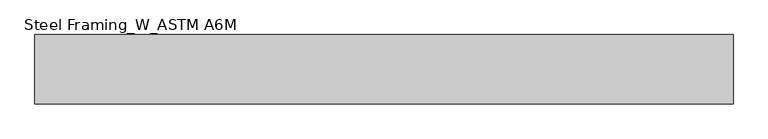
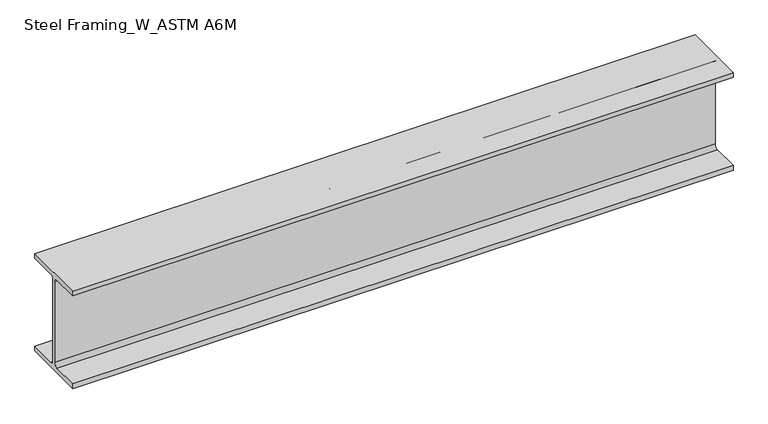
"""IFC4 building model written with IfcOpenShell, lengths in millimetres: beam geometry, Steel Framing_W_ASTM A6M : H_SB_AR_S02_W200x31.3_B6."""

from ifc_helpers import new_model, si_unit, point, frame, frame_2d, origin, place, context, project, spatial, polyline, circle_curve, trimmed, segment, composite_curve, outline, extrude, source, transform, mapped, element, save


def steel_framing_w_astm_a6m_deedff07(model_context):
    return source(origin(), model_context, "Body", "SweptSolid", [
        extrude(outline(composite_curve([segment(polyline([(67.0, -94.8), (67.0, -105.0), (-67.0, -105.0), (-67.0, -94.8), (-10.775, -94.8)]), True, "CONTINUOUS"), segment(trimmed(circle_curve(frame_2d((-10.775, -87.2)), 7.6), [point((-10.775, -94.8))], [point((-3.175, -87.2))], True, "CARTESIAN"), True, "CONTINUOUS"), segment(polyline([(-3.175, -87.2), (-3.175, 87.2)]), True, "CONTINUOUS"), segment(trimmed(circle_curve(frame_2d((-10.775, 87.2)), 7.6), [point((-3.175, 87.2))], [point((-10.775, 94.8))], True, "CARTESIAN"), True, "CONTINUOUS"), segment(polyline([(-10.775, 94.8), (-67.0, 94.8), (-67.0, 105.0), (67.0, 105.0), (67.0, 94.8), (10.775, 94.8)]), True, "CONTINUOUS"), segment(trimmed(circle_curve(frame_2d((10.775, 87.2)), 7.6), [point((10.775, 94.8))], [point((3.175, 87.2))], True, "CARTESIAN"), True, "CONTINUOUS"), segment(polyline([(3.175, 87.2), (3.175, -87.2)]), True, "CONTINUOUS"), segment(trimmed(circle_curve(frame_2d((10.775, -87.2)), 7.6), [point((3.175, -87.2))], [point((10.775, -94.8))], True, "CARTESIAN"), True, "CONTINUOUS"), segment(polyline([(10.775, -94.8), (67.0, -94.8)]), True, "CONTINUOUS")], self_intersect=False)), frame((-625.5, 0.0, 0.0), z_axis=(1.0, 0.0, 0.0), x_axis=(0.0, 1.0, 0.0)), (0.0, 0.0, 1.0), 1345.8),
    ])


if __name__ == "__main__":
    model = new_model("IFC4")
    model_context = context("Model", 3, world=origin())
    ifc_project = project(units=[si_unit("LENGTHUNIT", "METRE", prefix="MILLI")], contexts=[model_context])
    site = spatial("IfcSite", under=ifc_project)
    building = spatial("IfcBuilding", under=site)
    placement = place(None, origin())
    steel_framing_w_astm_a6m_shape = steel_framing_w_astm_a6m_deedff07(model_context)
    element("IfcBeam", 1, ObjectType="Steel Framing_W_ASTM A6M : H_SB_AR_S02_W200x31.3_B6", at=placement, inside=building, context=model_context, shape_type="MappedRepresentation", body=[
        mapped(steel_framing_w_astm_a6m_shape, transform((0.0, 0.0, 0.0), x_axis=(1.0, 0.0, 0.0), y_axis=(0.0, 1.0, 0.0), z_axis=(0.0, 0.0, 1.0))),
    ])
    save(model, "model.ifc")

# Revit data of these elements
# Type "Steel Framing_W_ASTM A6M : H_SB_AR_S02_W200x31.3_B6"
#   Type Mark = "B6"
#   Section Name Key = "W8x21"
#   Width = 13.4 cm
#   Web Thickness = 0.635 cm
#   Web Fillet = 0.76 cm
#   Warping Constant = 40800.0 cm⁶
#   Torsional Moment of Inertia = 11.70 cm⁴
#   Section Area = 39.7 cm²
#   Plastic Modulus weak axis = 93.2 cm³
#   Plastic Modulus strong axis = 334.0 cm³
#   Perimeter = 0.93 m²/m
#   Nominal Weight = 31.30 kgf/m
#   Moment of Inertia weak axis = 407.00 cm⁴
#   Moment of Inertia strong axis = 3130.00 cm⁴
#   Height = 21.0 cm
#   Flange Thickness = 1.02 cm
#   Elastic Modulus weak axis = 60.8 cm³
#   Elastic Modulus strong axis = 298.0 cm³
#   Centroid Vertical = 10.5 cm
#   Centroid Horizontal = 6.7 cm
#   Length [instance default] = 1500 mm
#   Structural Material [instance default] = Steel, 45-345
#   Bolt Spacing = 0
#   Assembly Code = ""
# Element 1 (IfcBeam, "Steel Framing_W_ASTM A6M : H_SB_AR_S02_W200x31.3_B6")
#   Materials on its faces: "Steel, 45-345"
# Materials
#   "Steel, 45-345": class "Metal", colour RGB 189 187 185, transparency 0, Description = "Steel 345 MPa", Cost = 0
